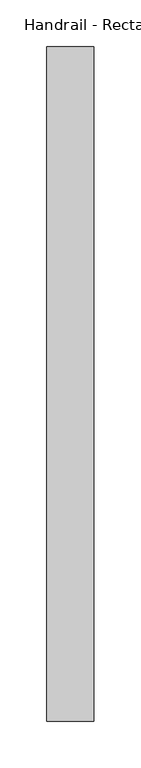
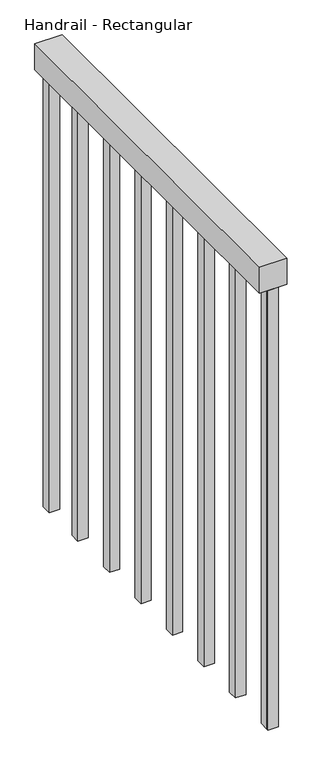
"""IFC4 building model written with IfcOpenShell, lengths in millimetres: railing geometry, Handrail - Rectangular."""

from ifc_helpers import new_model, si_unit, frame, origin, place, context, project, spatial, polyline, outline, extrude, source, transform, mapped, element, save


def handrail_rectangular_8194ed1a(model_context):
    return source(origin(), model_context, "Body", "SweptSolid", [
        extrude(outline(polyline([(-74561.7, 12852.4), (-74510.9, 12852.4), (-74510.9, 12128.5), (-74561.7, 12128.5), (-74561.7, 12852.4)])), frame((0.0, 0.0, 13430.25), z_axis=(0.0, 0.0, 1.0), x_axis=(1.0, 0.0, 0.0)), (0.0, 0.0, 1.0), 50.8),
        extrude(outline(polyline([(-74545.825, 12150.725), (-74526.775, 12150.725), (-74526.775, 12131.675), (-74545.825, 12131.675), (-74545.825, 12150.725)])), frame((0.0, 0.0, 12566.65), z_axis=(0.0, 0.0, 1.0), x_axis=(1.0, 0.0, 0.0)), (0.0, 0.0, 1.0), 863.6),
        extrude(outline(polyline([(-74545.825, 12252.325), (-74526.775, 12252.325), (-74526.775, 12233.275), (-74545.825, 12233.275), (-74545.825, 12252.325)])), frame((0.0, 0.0, 12566.65), z_axis=(0.0, 0.0, 1.0), x_axis=(1.0, 0.0, 0.0)), (0.0, 0.0, 1.0), 863.6),
        extrude(outline(polyline([(-74545.825, 12353.925), (-74526.775, 12353.925), (-74526.775, 12334.875), (-74545.825, 12334.875), (-74545.825, 12353.925)])), frame((0.0, 0.0, 12566.65), z_axis=(0.0, 0.0, 1.0), x_axis=(1.0, 0.0, 0.0)), (0.0, 0.0, 1.0), 863.6),
        extrude(outline(polyline([(-74545.825, 12455.525), (-74526.775, 12455.525), (-74526.775, 12436.475), (-74545.825, 12436.475), (-74545.825, 12455.525)])), frame((0.0, 0.0, 12566.65), z_axis=(0.0, 0.0, 1.0), x_axis=(1.0, 0.0, 0.0)), (0.0, 0.0, 1.0), 863.6),
        extrude(outline(polyline([(-74545.825, 12557.125), (-74526.775, 12557.125), (-74526.775, 12538.075), (-74545.825, 12538.075), (-74545.825, 12557.125)])), frame((0.0, 0.0, 12566.65), z_axis=(0.0, 0.0, 1.0), x_axis=(1.0, 0.0, 0.0)), (0.0, 0.0, 1.0), 863.6),
        extrude(outline(polyline([(-74545.825, 12658.725), (-74526.775, 12658.725), (-74526.775, 12639.675), (-74545.825, 12639.675), (-74545.825, 12658.725)])), frame((0.0, 0.0, 12566.65), z_axis=(0.0, 0.0, 1.0), x_axis=(1.0, 0.0, 0.0)), (0.0, 0.0, 1.0), 863.6),
        extrude(outline(polyline([(-74545.825, 12760.325), (-74526.775, 12760.325), (-74526.775, 12741.275), (-74545.825, 12741.275), (-74545.825, 12760.325)])), frame((0.0, 0.0, 12566.65), z_axis=(0.0, 0.0, 1.0), x_axis=(1.0, 0.0, 0.0)), (0.0, 0.0, 1.0), 863.6),
        extrude(outline(polyline([(-74545.825, 12147.55), (-74526.775, 12147.55), (-74526.775, 12128.5), (-74545.825, 12128.5), (-74545.825, 12147.55)])), frame((0.0, 0.0, 12566.65), z_axis=(0.0, 0.0, 1.0), x_axis=(1.0, 0.0, 0.0)), (0.0, 0.0, 1.0), 863.6),
        extrude(outline(polyline([(-74545.825, 12852.4), (-74526.775, 12852.4), (-74526.775, 12833.35), (-74545.825, 12833.35), (-74545.825, 12852.4)])), frame((0.0, 0.0, 12566.65), z_axis=(0.0, 0.0, 1.0), x_axis=(1.0, 0.0, 0.0)), (0.0, 0.0, 1.0), 863.6),
    ])


if __name__ == "__main__":
    model = new_model("IFC4")
    model_context = context("Model", 3, world=origin())
    ifc_project = project(units=[si_unit("LENGTHUNIT", "METRE", prefix="MILLI")], contexts=[model_context])
    site = spatial("IfcSite", under=ifc_project)
    building = spatial("IfcBuilding", under=site)
    placement = place(None, origin())
    handrail_rectangular_shape = handrail_rectangular_8194ed1a(model_context)
    element("IfcRailing", 1, ObjectType="Handrail - Rectangular", at=placement, inside=building, context=model_context, shape_type="MappedRepresentation", body=[
        mapped(handrail_rectangular_shape, transform((0.0, 0.0, 0.0), x_axis=(1.0, 0.0, 0.0), y_axis=(0.0, 1.0, 0.0), z_axis=(0.0, 0.0, 1.0))),
    ])
    save(model, "model.ifc")
